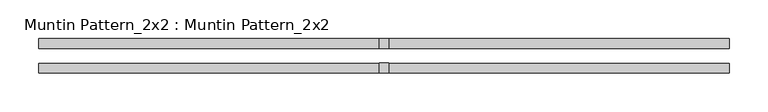
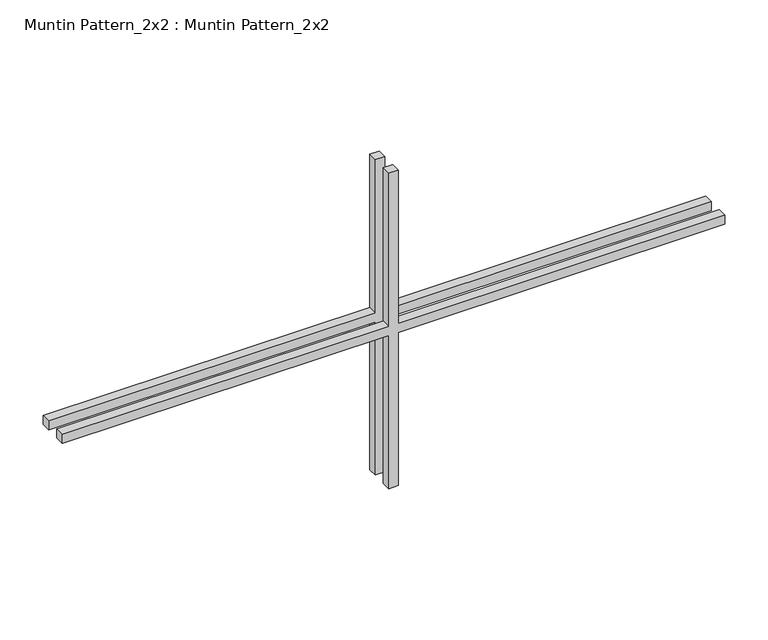
"""IFC4 building model written with IfcOpenShell, lengths in millimetres: proxy geometry, Muntin Pattern_2x2 : Muntin Pattern_2x2."""

from ifc_helpers import new_model, si_unit, frame, origin, place, context, project, spatial, polyline, outline, extrude, source, transform, mapped, element, save


def muntin_pattern_2x2_muntin_pattern_2x2_39bd07d8(model_context):
    return source(origin(), model_context, "Body", "SweptSolid", [
        extrude(outline(polyline([(230.1875, -6.35), (230.1875, -444.5), (217.4875, -444.5), (217.4875, -6.35), (0.0, -6.35), (0.0, 6.35), (217.4875, 6.35), (217.4875, 444.5), (230.1875, 444.5), (230.1875, 6.35), (447.675, 6.35), (447.675, -6.35), (230.1875, -6.35)])), frame((0.0, -22.225, 0.0), z_axis=(0.0, 1.0, 0.0), x_axis=(0.0, 0.0, 1.0)), (0.0, 0.0, 1.0), 12.7),
        extrude(outline(polyline([(230.1875, -6.35), (230.1875, -444.5), (217.4875, -444.5), (217.4875, -6.35), (0.0, -6.35), (0.0, 6.35), (217.4875, 6.35), (217.4875, 444.5), (230.1875, 444.5), (230.1875, 6.35), (447.675, 6.35), (447.675, -6.35), (230.1875, -6.35)])), frame((0.0, 9.525, 0.0), z_axis=(0.0, 1.0, 0.0), x_axis=(0.0, 0.0, 1.0)), (0.0, 0.0, 1.0), 12.7),
    ])


if __name__ == "__main__":
    model = new_model("IFC4")
    model_context = context("Model", 3, world=origin())
    ifc_project = project(units=[si_unit("LENGTHUNIT", "METRE", prefix="MILLI")], contexts=[model_context])
    site = spatial("IfcSite", under=ifc_project)
    building = spatial("IfcBuilding", under=site)
    placement = place(None, origin())
    muntin_pattern_2x2_muntin_pattern_2x2_shape = muntin_pattern_2x2_muntin_pattern_2x2_39bd07d8(model_context)
    element("IfcBuildingElementProxy", 1, Name="Muntin Pattern_2x2 : Muntin Pattern_2x2", ObjectType="Muntin Pattern_2x2 : Muntin Pattern_2x2", at=placement, inside=building, context=model_context, shape_type="MappedRepresentation", body=[
        mapped(muntin_pattern_2x2_muntin_pattern_2x2_shape, transform((0.0, 0.0, 0.0), x_axis=(1.0, 0.0, 0.0), y_axis=(0.0, 1.0, 0.0), z_axis=(0.0, 0.0, 1.0))),
    ])
    save(model, "model.ifc")

# Revit data of these elements
# Type "Muntin Pattern_2x2 : Muntin Pattern_2x2"
#   Width [instance default] = 4' - 0"
#   Thickness = 0' - 0 1/2"
#   Height [instance default] = 4' - 0"
#   Distance = 0' - 0 3/4"
#   Interior Material [instance default] = none
#   Exterior Material [instance default] = none
# Element 1 (IfcBuildingElementProxy, "Muntin Pattern_2x2 : Muntin Pattern_2x2")
#   Width = 2' - 11"
#   Height = 1' - 5 5/8"
#   Interior Material = Wood - Stained
#   Exterior Material = Clad - White
#   Materials on its faces: "Clad - White", "Wood - Stained"
# Materials
#   "Clad - White": class "Wood", colour RGB 242 242 238, transparency 0, Cost = 0
#   "Wood - Stained": class "Wood", colour RGB 224 178 126, transparency 0, Cost = 0
